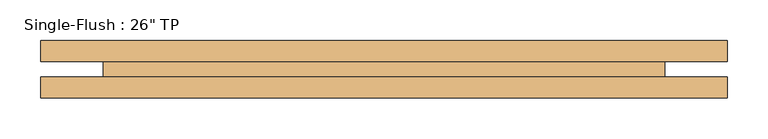
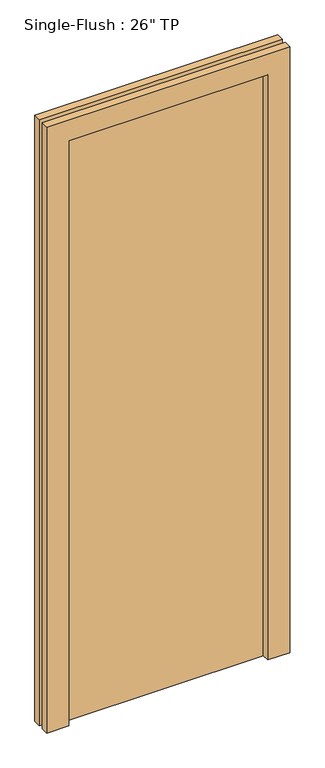
"""IFC4 building model written with IfcOpenShell, lengths in millimetres: door geometry."""

from ifc_helpers import new_model, si_unit, frame, origin, origin_with_axes, place, context, project, spatial, polyline, outline, extrude, source, transform, mapped, element, save


def door_b9e9bd48(model_context):
    return source(origin(), model_context, "Body", "SweptSolid", [
        extrude(outline(polyline([(2209.8, -419.1), (0.0, -419.1), (0.0, -342.9), (2133.6, -342.9), (2133.6, 342.9), (0.0, 342.9), (0.0, 419.1), (2209.8, 419.1), (2209.8, -419.1)])), frame((0.0, -34.925, 0.0), z_axis=(0.0, 1.0, 0.0), x_axis=(0.0, 0.0, 1.0)), (0.0, 0.0, 1.0), 25.4),
        extrude(outline(polyline([(2209.8, 419.1), (2209.8, -419.1), (0.0, -419.1), (0.0, -342.9), (2133.6, -342.9), (2133.6, 342.9), (0.0, 342.9), (0.0, 419.1), (2209.8, 419.1)])), frame((0.0, 9.525, 0.0), z_axis=(0.0, 1.0, 0.0), x_axis=(0.0, 0.0, 1.0)), (0.0, 0.0, 1.0), 25.4),
        extrude(outline(polyline([(342.9, 9.525), (342.9, -9.525), (-342.9, -9.525), (-342.9, 9.525), (342.9, 9.525)])), origin_with_axes(), (0.0, 0.0, 1.0), 2133.6),
    ])


if __name__ == "__main__":
    model = new_model("IFC4")
    model_context = context("Model", 3, world=origin())
    ifc_project = project(units=[si_unit("LENGTHUNIT", "METRE", prefix="MILLI")], contexts=[model_context])
    site = spatial("IfcSite", under=ifc_project)
    building = spatial("IfcBuilding", under=site)
    placement = place(None, origin())
    door_shape = door_b9e9bd48(model_context)
    element("IfcDoor", 1, ObjectType="Single-Flush : 26\" TP", at=placement, inside=building, context=model_context, shape_type="MappedRepresentation", body=[
        mapped(door_shape, transform((0.0, 0.0, 0.0), x_axis=(1.0, 0.0, 0.0), y_axis=(0.0, 1.0, 0.0), z_axis=(0.0, 0.0, 1.0))),
    ])
    save(model, "model.ifc")

# Revit data of these elements
# Type "Single-Flush : 26\" TP"
#   Type Mark = "56"
#   Construction Type Id = "MDOOR"
#   Assembly Code = "C1020"
#   Analytic Construction = "Metal"
#   Thickness = 0' - 0 3/4"
#   Heat Transfer Coefficient (U) = 3.7021 W/(m²·K)
#   Height = 7' - 0"
#   Trim Projection Ext = 0' - 1"
#   Trim Projection Int = 0' - 1"
#   Trim Width = 0' - 3"
#   Width = 2' - 3"
#   Door Material = Door - Panel
#   Frame Material = Door - Frame
#   Visual Light Transmittance = 0
#   Solar Heat Gain Coefficient = 0
#   Function = (empty or 0)
#   Wall Closure = (empty or 0)
# Element 1 (IfcDoor, "Single-Flush : 26\" TP")
#   Materials on its faces: "Door - Frame", "Door - Panel"
# Materials
#   "Door - Panel": class "Wood", colour RGB 210 159 95, transparency 0
#   "Door - Frame": class "Miscellaneous", colour RGB 118 70 51, transparency 0
